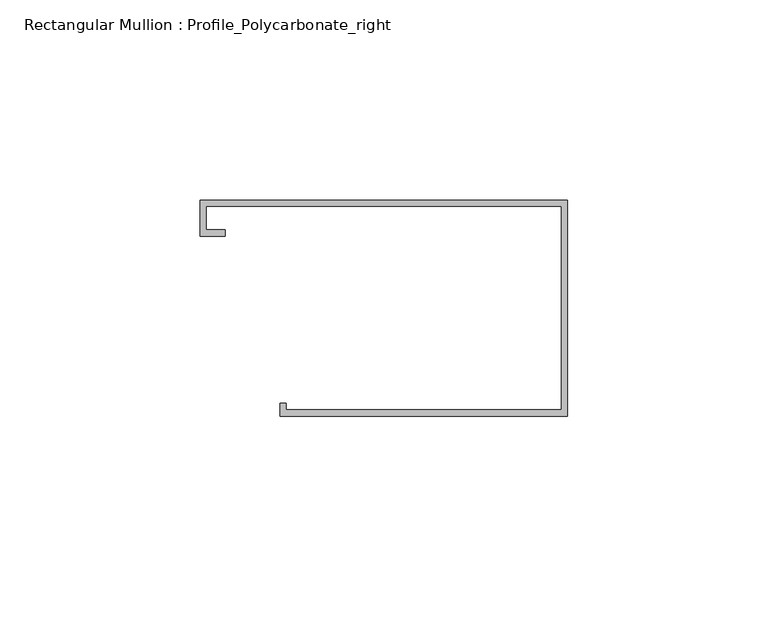
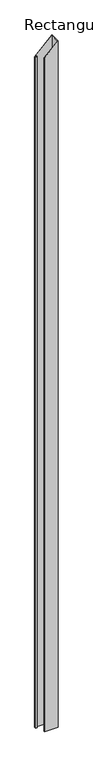
"""IFC4 building model written with IfcOpenShell, lengths in millimetres: member geometry, Rectangular Mullion : Profile_Polycarbonate_right."""

from ifc_helpers import new_model, si_unit, origin, place, context, project, spatial, faceted_brep, source, transform, mapped, element, save


def rectangular_mullion_profile_polycarbonate_right_87805b23(model_context):
    return source(origin(), model_context, "Body", "Brep", [
        faceted_brep([(0.0, 28.984575, -3799.7325811), (0.0, -25.015825, -3799.7325811), (-71.9836, -25.015825, -3799.7325811), (-71.9836, -21.840825, -3799.7325811), (-70.3961, -21.840825, -3799.7325811), (-70.3961, -23.428325, -3799.7325811), (-1.5875, -23.428325, -3799.7325811), (-1.5875, 27.397075, -3799.7325811), (-90.4113, 27.397075, -3799.7325811), (-90.4113, 21.580475, -3799.7325811), (-85.6488, 21.580475, -3799.7325811), (-85.6488, 19.992975, -3799.7325811), (-91.9988, 19.992975, -3799.7325811), (-91.9988, 28.984575, -3799.7325811), (-91.9988, 28.984575, -88.2453421), (0.0, 28.984575, 0.0), (-91.9988, 19.992975, -88.2453421), (-85.6488, 19.992975, -82.1544157), (-85.6488, 21.580475, -82.1544157), (-90.4113, 21.580475, -86.7226105), (-90.4113, 27.397075, -86.7226105), (-1.5875, 27.397075, -1.5227316), (-1.5875, -23.428325, -1.5227316), (-70.3961, -23.428325, -67.5240104), (-70.3961, -21.840825, -67.5240104), (-71.9836, -21.840825, -69.046742), (-71.9836, -25.015825, -69.046742), (0.0, -25.015825, 0.0)], [[[0, 1, 2, 3, 4, 5, 6, 7, 8, 9, 10, 11, 12, 13]], [[14, 15, 0, 13]], [[16, 14, 13, 12]], [[17, 16, 12, 11]], [[18, 17, 11, 10]], [[19, 18, 10, 9]], [[20, 19, 9, 8]], [[21, 20, 8, 7]], [[22, 21, 7, 6]], [[23, 22, 6, 5]], [[24, 23, 5, 4]], [[25, 24, 4, 3]], [[26, 25, 3, 2]], [[27, 26, 2, 1]], [[15, 27, 1, 0]], [[15, 14, 16, 17, 18, 19, 20, 21, 22, 23, 24, 25, 26, 27]]]),
    ])


if __name__ == "__main__":
    model = new_model("IFC4")
    model_context = context("Model", 3, world=origin())
    ifc_project = project(units=[si_unit("LENGTHUNIT", "METRE", prefix="MILLI")], contexts=[model_context])
    site = spatial("IfcSite", under=ifc_project)
    building = spatial("IfcBuilding", under=site)
    placement = place(None, origin())
    rectangular_mullion_profile_polycarbonate_right_shape = rectangular_mullion_profile_polycarbonate_right_87805b23(model_context)
    element("IfcMember", 1, ObjectType="Rectangular Mullion : Profile_Polycarbonate_right", at=placement, inside=building, context=model_context, shape_type="MappedRepresentation", body=[
        mapped(rectangular_mullion_profile_polycarbonate_right_shape, transform((0.0, 0.0, 0.0), x_axis=(1.0, 0.0, 0.0), y_axis=(0.0, 1.0, 0.0), z_axis=(0.0, 0.0, 1.0))),
    ])
    save(model, "model.ifc")

# Revit data of these elements
# Type "Rectangular Mullion : Profile_Polycarbonate_right"
#   built-in parameter 1007322 = 0.177167 (stored number, unit not read)
#   built-in parameter 1007321 = 0 (stored number, unit not read)
#   built-in parameter 1007320 = 0.00520833 (stored number, unit not read)
